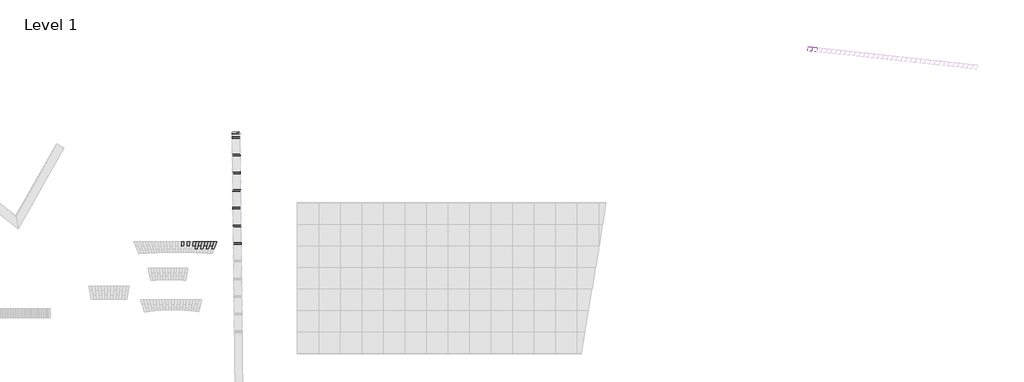
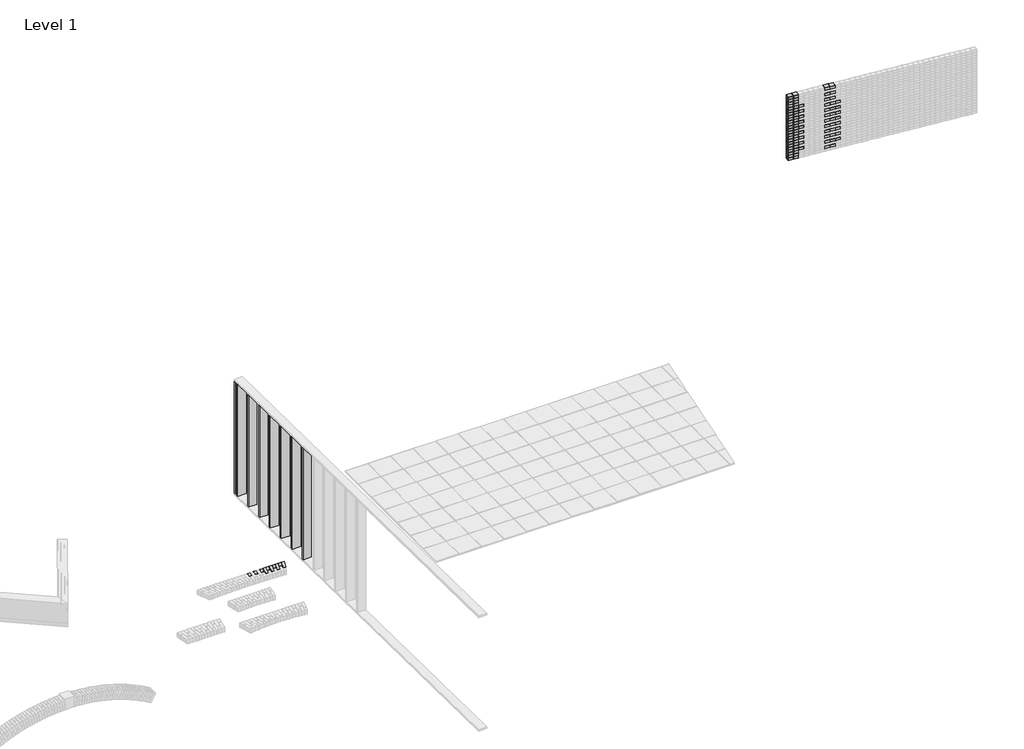
# One storey, part 11 of 18: 107 proxies.
"""IFC4 building model written with IfcOpenShell, lengths in millimetres."""

import ifcopenshell
import ifcopenshell.guid

model = None  # the IFC model being written
_history = None  # IfcOwnerHistory: only IFC2X3 demands one
_inside = {}  # id of a spatial element -> (the spatial element, [elements in it])
_under = {}  # id of a project, library or spatial element -> (it, [spatial elements below it])
_declared = {}  # id of a project -> (the project, [libraries it declares])
_typed = {}  # id of a type object -> (the type object, [elements of that type])
_made_of = {}  # id of a material, layer set ... -> (it, [elements and type objects made of it])


def new_model(schema):
    """Start an empty IFC model of exactly this schema.

    Asked for "IFC4X3", IfcOpenShell would pick the latest addendum, in which some entities
    have other attributes; the version numbers below select the first issue.
    IFC2X3 requires an IfcOwnerHistory on every rooted entity: one is made here for all.
    """
    global model, _history
    if schema == "IFC4X3":
        model = ifcopenshell.file(schema_version=(4, 3, 0, 0))
    else:
        model = ifcopenshell.file(schema=schema)
    _inside.clear()
    _under.clear()
    _declared.clear()
    _typed.clear()
    _made_of.clear()
    _history = None
    if model.schema == "IFC2X3":
        org = make("IfcOrganization", Name="unknown")
        user = make(
            "IfcPersonAndOrganization",
            ThePerson=make("IfcPerson", FamilyName="unknown"),
            TheOrganization=org,
        )
        app = make(
            "IfcApplication",
            ApplicationDeveloper=org,
            Version="unknown",
            ApplicationFullName="unknown",
            ApplicationIdentifier="unknown",
        )
        _history = make(
            "IfcOwnerHistory",
            OwningUser=user,
            OwningApplication=app,
            ChangeAction="ADDED",
            CreationDate=0,
        )
    return model


def make(cls, **values):
    """One entity of the class cls with the attributes given. An attribute that is None is left unset."""
    return model.create_entity(
        cls, **{name: value for name, value in values.items() if value is not None}
    )


def rooted(cls, **values):
    """An entity with a GlobalId (a new one), such as an element, a storey or a relation."""
    return make(cls, GlobalId=ifcopenshell.guid.new(), OwnerHistory=_history, **values)


def si_unit(unit_type, name, prefix=None):
    """IfcSIUnit, for example si_unit("LENGTHUNIT", "METRE", prefix="MILLI")."""
    return make("IfcSIUnit", UnitType=unit_type, Prefix=prefix, Name=name)


def assignment(units):
    """IfcUnitAssignment: the units of a project."""
    return None if units is None else make("IfcUnitAssignment", Units=units)


def point(xyz):
    """IfcCartesianPoint."""
    return None if xyz is None else make("IfcCartesianPoint", Coordinates=xyz)


def direction(xyz):
    """IfcDirection."""
    return None if xyz is None else make("IfcDirection", DirectionRatios=xyz)


def frame(location, z_axis=None, x_axis=None):
    """IfcAxis2Placement3D, a coordinate frame: its origin and axes. An axis left out is left unset."""
    return make(
        "IfcAxis2Placement3D",
        Location=point(location),
        Axis=direction(z_axis),
        RefDirection=direction(x_axis),
    )


def origin():
    """The frame at (0, 0, 0) with its axes left unset."""
    return frame((0.0, 0.0, 0.0))


def origin_with_axes():
    """The frame at (0, 0, 0) with the z axis (0, 0, 1) and the x axis (1, 0, 0) written out."""
    return frame((0.0, 0.0, 0.0), z_axis=(0.0, 0.0, 1.0), x_axis=(1.0, 0.0, 0.0))


def place(relative_to, where):
    """IfcLocalPlacement: puts the frame where relative to a parent placement (None: the world)."""
    return make(
        "IfcLocalPlacement", PlacementRelTo=relative_to, RelativePlacement=where
    )


def context(
    kind, dimensions, precision=None, world=None, true_north=None, identifier=None
):
    """IfcGeometricRepresentationContext, for example the 3D "Model" context."""
    return make(
        "IfcGeometricRepresentationContext",
        ContextIdentifier=identifier,
        ContextType=kind,
        CoordinateSpaceDimension=dimensions,
        Precision=precision,
        WorldCoordinateSystem=world,
        TrueNorth=true_north,
    )


def project(units=None, contexts=None):
    """IfcProject with its units and contexts."""
    return rooted(
        "IfcProject",
        Name="project",
        RepresentationContexts=contexts,
        UnitsInContext=assignment(units),
    )


def spatial(cls, under=None, at=None, **own):
    """A site, building, storey or space (cls), placed at a placement, below another one or the project."""
    s = rooted(cls, ObjectPlacement=at, **own)
    if under is not None:
        _under.setdefault(under.id(), (under, []))[1].append(s)
    return s


def polyline(points):
    """IfcPolyline through the points."""
    return make("IfcPolyline", Points=[point(p) for p in points])


def outline(outer, holes=None, kind="AREA"):
    """IfcArbitraryClosedProfileDef: a profile drawn as a closed curve; with holes, ...WithVoids."""
    if holes is None:
        return make("IfcArbitraryClosedProfileDef", ProfileType=kind, OuterCurve=outer)
    return make(
        "IfcArbitraryProfileDefWithVoids",
        ProfileType=kind,
        OuterCurve=outer,
        InnerCurves=holes,
    )


def extrude(swept, where, along, depth):
    """IfcExtrudedAreaSolid: the profile swept, set in the frame where, extruded along a direction by depth."""
    return make(
        "IfcExtrudedAreaSolid",
        SweptArea=swept,
        Position=where,
        ExtrudedDirection=direction(along),
        Depth=depth,
    )


def shape(context_of_items, identifier, shape_type, items):
    """IfcShapeRepresentation: the items that make up one representation, for example the "Body"."""
    return make(
        "IfcShapeRepresentation",
        ContextOfItems=context_of_items,
        RepresentationIdentifier=identifier,
        RepresentationType=shape_type,
        Items=items,
    )


def source(mapping_origin, context_of_items, identifier, shape_type, items):
    """IfcRepresentationMap: a shape defined once, which mapped items show again and again."""
    return make(
        "IfcRepresentationMap",
        MappingOrigin=mapping_origin,
        MappedRepresentation=shape(context_of_items, identifier, shape_type, items),
    )


def transform(
    local_origin,
    x_axis=None,
    y_axis=None,
    z_axis=None,
    scale=None,
    scale2=None,
    scale3=None,
    uniform=True,
):
    """IfcCartesianTransformationOperator3D, or its non-uniform kind. x_axis, y_axis, z_axis: its Axis1, 2, 3."""
    if uniform:
        return make(
            "IfcCartesianTransformationOperator3D",
            Axis1=direction(x_axis),
            Axis2=direction(y_axis),
            LocalOrigin=point(local_origin),
            Scale=scale,
            Axis3=direction(z_axis),
        )
    return make(
        "IfcCartesianTransformationOperator3DnonUniform",
        Axis1=direction(x_axis),
        Axis2=direction(y_axis),
        LocalOrigin=point(local_origin),
        Scale=scale,
        Axis3=direction(z_axis),
        Scale2=scale2,
        Scale3=scale3,
    )


def mapped(mapping_source, mapping_target):
    """IfcMappedItem: shows the shape of a source again, moved by a transform."""
    return make(
        "IfcMappedItem", MappingSource=mapping_source, MappingTarget=mapping_target
    )


def made_of(thing, what):
    """Note that an element or type object is made of a material, layer set ...; save() writes the relation."""
    if what is not None:
        _made_of.setdefault(what.id(), (what, []))[1].append(thing)
    return thing


def element(
    cls,
    number,
    at=None,
    inside=None,
    cuts=None,
    type_object=None,
    material=None,
    context=None,
    identifier="Body",
    shape_type=None,
    held_by="IfcProductDefinitionShape",
    body=None,
    shapes=None,
    **own,
):
    """One element of the class cls, such as IfcWall. Its Tag is "e" and its number.

    at: its placement. inside: the storey or other place that contains it. cuts: it is an
    opening in that element (IfcRelVoidsElement). A single representation is given by context,
    identifier, shape_type and body (its items); several are given by shapes. held_by: the class
    of the entity that holds the representations. save() writes the other relations.
    """
    e = rooted(cls, Tag="e%d" % number, ObjectPlacement=at, **own)
    if body is not None:
        shapes = [shape(context, identifier, shape_type, body)]
    if shapes is not None:
        e.Representation = make(held_by, Representations=shapes)
    if inside is not None:
        _inside.setdefault(inside.id(), (inside, []))[1].append(e)
    if cuts is not None:
        rooted(
            "IfcRelVoidsElement", RelatingBuildingElement=cuts, RelatedOpeningElement=e
        )
    if type_object is not None:
        _typed.setdefault(type_object.id(), (type_object, []))[1].append(e)
    return made_of(e, material)


def aggregate(whole, parts):
    """IfcRelAggregates: a whole, such as a stair, and the parts it consists of."""
    return rooted("IfcRelAggregates", RelatingObject=whole, RelatedObjects=parts)


def save(model, path):
    """Write the relations noted so far, then the file.

    IfcRelAggregates (storeys below a building ...), IfcRelContainedInSpatialStructure (elements
    in a storey), IfcRelDefinesByType, IfcRelAssociatesMaterial and IfcRelDeclares: one each for
    every whole, place, type object, material and project.
    """
    for whole, parts in _under.values():
        aggregate(whole, parts)
    for where, things in _inside.values():
        rooted(
            "IfcRelContainedInSpatialStructure",
            RelatedElements=things,
            RelatingStructure=where,
        )
    for kind, things in _typed.values():
        rooted("IfcRelDefinesByType", RelatedObjects=things, RelatingType=kind)
    for what, things in _made_of.values():
        rooted("IfcRelAssociatesMaterial", RelatedObjects=things, RelatingMaterial=what)
    for by, libraries in _declared.values():
        rooted("IfcRelDeclares", RelatingContext=by, RelatedDefinitions=libraries)
    model.write(path)


def proxy_00_gma_hout_184x38_1d2382f2(model_context):
    return source(origin(), model_context, "Body", "SweptSolid", [
        extrude(outline(polyline([(-19.0, 0.0), (19.0, 0.0), (19.0, -2617.0000001), (-19.0, -2617.0000001), (-19.0, 0.0)])), frame((-400.2270235, 19.0, -613.6855812), z_axis=(-0.67357883778224, 0.0, 0.7391153829355245), x_axis=(0.0, 1.0, 0.0)), (0.0, 0.0, 1.0), 184.0),
    ])


def proxy_00_gma_hout_38x184_71ec18f3(model_context):
    return source(origin(), model_context, "Body", "SweptSolid", [
        extrude(outline(polyline([(-19.0, 0.0), (19.0, 0.0), (19.0, -2617.0000001), (-19.0, -2617.0000001), (-19.0, 0.0)])), frame((-400.2270235, 19.0, -613.6855812), z_axis=(-0.6735788377822399, 0.0, 0.7391153829355245), x_axis=(0.0, 1.0, 0.0)), (0.0, 0.0, 1.0), 184.0),
    ])


def geel_a5fc7152(model_context):
    return source(origin(), model_context, "Body", "SweptSolid", [
        extrude(outline(polyline([(131.1871262, 51.8695461), (24.8461542, 24.0369432), (23.5801491, 28.8740117), (125.0840527, 55.4406095), (111.9430518, 105.6488784), (10.4391482, 79.0822806), (9.1731432, 83.919349), (115.5141152, 111.7519519), (131.1871262, 51.8695461)])), origin_with_axes(), (0.0, 0.0, 1.0), 95.0),
        extrude(outline(polyline([(111.9430518, 105.6488784), (125.0840527, 55.4406095), (23.5801491, 28.8740117), (10.4391482, 79.0822806), (111.9430518, 105.6488784)])), origin_with_axes(), (0.0, 0.0, 1.0), 100.0),
    ])


def geel_ff5a4212(model_context):
    return source(origin(), model_context, "Body", "SweptSolid", [
        extrude(outline(polyline([(24.8461542, 24.0369432), (9.1731432, 83.919349), (115.5141152, 111.7519519), (116.7801202, 106.9148835), (15.2762167, 80.3482856), (28.4172176, 30.1400167), (129.9211211, 56.7066146), (131.1871262, 51.8695461), (24.8461542, 24.0369432)])), origin_with_axes(), (0.0, 0.0, 1.0), 95.0),
        extrude(outline(polyline([(116.7801202, 106.9148835), (129.9211211, 56.7066146), (28.4172176, 30.1400167), (15.2762167, 80.3482856), (116.7801202, 106.9148835)])), origin_with_axes(), (0.0, 0.0, 1.0), 100.0),
    ])


def rood_14a66368(model_context):
    return source(origin(), model_context, "Body", "SweptSolid", [
        extrude(outline(polyline([(24.8461542, 24.0369432), (9.1731432, 83.919349), (115.5141152, 111.7519519), (131.1871262, 51.8695461), (24.8461542, 24.0369432)]), holes=[polyline([(125.0840527, 55.4406095), (111.9430518, 105.6488784), (15.2762167, 80.3482856), (28.4172176, 30.1400167), (125.0840527, 55.4406095)])]), origin_with_axes(), (0.0, 0.0, 1.0), 95.0),
        extrude(outline(polyline([(111.9430518, 105.6488784), (125.0840527, 55.4406095), (28.4172176, 30.1400167), (15.2762167, 80.3482856), (111.9430518, 105.6488784)])), origin_with_axes(), (0.0, 0.0, 1.0), 100.0),
    ])


def steen_boven_01e32946(model_context):
    return source(origin(), model_context, "Body", "SweptSolid", [
        extrude(outline(polyline([(141.1704134, 152.36343), (62.4529027, -8.187695), (10.0350866, 5.3211774), (84.0648392, 167.0564768), (141.1704134, 152.36343)])), origin_with_axes(), (0.0, 0.0, 1.0), 100.0),
    ])


def steen_boven_6e46f58c(model_context):
    return source(origin(), model_context, "Body", "SweptSolid", [
        extrude(outline(polyline([(143.5582911, 152.2686047), (60.0999612, -8.4277022), (7.3163998, 3.5526856), (86.0489792, 165.2920935), (143.5582911, 152.2686047)])), origin_with_axes(), (0.0, 0.0, 1.0), 100.0),
    ])


def steen_boven_eabcd001(model_context):
    return source(origin(), model_context, "Body", "SweptSolid", [
        extrude(outline(polyline([(146.1086958, 152.321622), (57.5952589, -8.8049317), (4.5075261, 1.71935), (88.2622432, 163.7549131), (146.1086958, 152.321622)])), origin_with_axes(), (0.0, 0.0, 1.0), 100.0),
    ])


def steen_boven_7310186c(model_context):
    return source(origin(), model_context, "Body", "SweptSolid", [
        extrude(outline(polyline([(148.8055175, 152.5156886), (54.9522509, -9.3122663), (1.614426, -0.1736166), (90.6804944, 162.4360672), (148.8055175, 152.5156886)])), origin_with_axes(), (0.0, 0.0, 1.0), 100.0),
    ])


def steen_boven_9bb71775(model_context):
    return source(origin(), model_context, "Body", "SweptSolid", [
        extrude(outline(polyline([(111.9849233, 118.6347443), (90.2344792, 23.3760955), (33.8999775, 23.0709028), (53.0204132, 118.2901143), (111.9849233, 118.6347443)])), origin_with_axes(), (0.0, 0.0, 1.0), 100.0),
    ])


def steen_boven_9cbfec4d(model_context):
    return source(origin(), model_context, "Body", "SweptSolid", [
        extrude(outline(polyline([(113.9568566, 118.7889283), (88.4390091, 23.0223042), (32.1209988, 21.8380681), (55.0050159, 117.5190081), (113.9568566, 118.7889283)])), origin_with_axes(), (0.0, 0.0, 1.0), 100.0),
    ])


def steen_boven_ecc8bb5a(model_context):
    return source(origin(), model_context, "Body", "SweptSolid", [
        extrude(outline(polyline([(115.9629985, 119.0094516), (86.6063002, 22.6045748), (30.3176515, 20.5836998), (57.0367025, 116.8591339), (115.9629985, 119.0094516)])), origin_with_axes(), (0.0, 0.0, 1.0), 100.0),
    ])


def steen_boven_26140218(model_context):
    return source(origin(), model_context, "Body", "SweptSolid", [
        extrude(outline(polyline([(106.3172402, 118.6145349), (95.374274, 24.0083503), (39.0907656, 26.6225769), (47.4149135, 121.3436608), (106.3172402, 118.6145349)])), origin_with_axes(), (0.0, 0.0, 1.0), 100.0),
    ])


def steen_boven_4abb9939(model_context):
    return source(origin(), model_context, "Body", "SweptSolid", [
        extrude(outline(polyline([(108.1602922, 118.5428629), (93.704652, 23.8737179), (37.3847868, 25.4648208), (49.2179184, 120.1947689), (108.1602922, 118.5428629)])), origin_with_axes(), (0.0, 0.0, 1.0), 100.0),
    ])


def steen_boven_6d657369(model_context):
    return source(origin(), model_context, "Body", "SweptSolid", [
        extrude(outline(polyline([(110.0512234, 118.5512029), (91.9904937, 23.66143), (35.6545533, 24.2803953), (51.0890541, 119.1795406), (110.0512234, 118.5512029)])), origin_with_axes(), (0.0, 0.0, 1.0), 100.0),
    ])


model = new_model("IFC4")

# Units and contexts
model_context = context("Model", 3, world=origin())
ifc_project = project(units=[si_unit("LENGTHUNIT", "METRE", prefix="MILLI")], contexts=[model_context])

# Site, building, storey
site = spatial("IfcSite", under=ifc_project)
building = spatial("IfcBuilding", under=site)
storey = spatial("IfcBuildingStorey", under=building, Name="Level 1", Elevation=0.0)

# Proxies
placement = place(None, origin())
proxy_00_gma_hout_184x38_shape = proxy_00_gma_hout_184x38_1d2382f2(model_context)
element("IfcBuildingElementProxy", 1, Name="00_GMA_hout : 184x38", ObjectType="00_GMA_hout : 184x38", at=placement, inside=storey, context=model_context, shape_type="MappedRepresentation", body=[
    mapped(proxy_00_gma_hout_184x38_shape, transform((-4279.0312737, -6270.7891061, 754.1795702), x_axis=(-0.6735355593090224, -0.007635512710727629, 0.7391153829355245), y_axis=(0.011335737232879188, -0.9999357484665639, 0.0), z_axis=(0.7390678936387847, 0.008378417765735984, 0.67357883778224))),
])
proxy_00_gma_hout_38x184_shape = proxy_00_gma_hout_38x184_71ec18f3(model_context)
element("IfcBuildingElementProxy", 2, Name="00_GMA_hout : 38x184", ObjectType="00_GMA_hout : 38x184", at=placement, inside=storey, context=model_context, shape_type="MappedRepresentation", body=[
    mapped(proxy_00_gma_hout_38x184_shape, transform((-4250.0117864, -8830.6246222, 754.1795702), x_axis=(-0.6735355593090224, -0.007635512710727629, 0.7391153829355245), y_axis=(0.011335737232879188, -0.9999357484665639, 0.0), z_axis=(0.7390678936387847, 0.008378417765735984, 0.67357883778224))),
])
element("IfcBuildingElementProxy", 3, Name="00_GMA_hout : 38x184", ObjectType="00_GMA_hout : 38x184", at=placement, inside=storey, context=model_context, shape_type="MappedRepresentation", body=[
    mapped(proxy_00_gma_hout_38x184_shape, transform((-4254.6594386, -8420.6509653, 754.1795702), x_axis=(-0.6735355593090224, -0.007635512710727629, 0.7391153829355245), y_axis=(0.011335737232879188, -0.9999357484665639, 0.0), z_axis=(0.7390678936387847, 0.008378417765735984, 0.67357883778224))),
])
element("IfcBuildingElementProxy", 4, Name="00_GMA_hout : 38x184", ObjectType="00_GMA_hout : 38x184", at=placement, inside=storey, context=model_context, shape_type="MappedRepresentation", body=[
    mapped(proxy_00_gma_hout_38x184_shape, transform((-4259.3070909, -8010.6773084, 754.1795702), x_axis=(-0.6735355593090224, -0.007635512710727629, 0.7391153829355245), y_axis=(0.011335737232879188, -0.9999357484665639, 0.0), z_axis=(0.7390678936387847, 0.008378417765735984, 0.67357883778224))),
])
element("IfcBuildingElementProxy", 5, Name="00_GMA_hout : 38x184", ObjectType="00_GMA_hout : 38x184", at=placement, inside=storey, context=model_context, shape_type="MappedRepresentation", body=[
    mapped(proxy_00_gma_hout_38x184_shape, transform((-4263.9547432, -7600.7036515, 754.1795702), x_axis=(-0.6735355593090224, -0.007635512710727629, 0.7391153829355245), y_axis=(0.011335737232879188, -0.9999357484665639, 0.0), z_axis=(0.7390678936387847, 0.008378417765735984, 0.67357883778224))),
])
element("IfcBuildingElementProxy", 6, Name="00_GMA_hout : 38x184", ObjectType="00_GMA_hout : 38x184", at=placement, inside=storey, context=model_context, shape_type="MappedRepresentation", body=[
    mapped(proxy_00_gma_hout_38x184_shape, transform((-4268.6023954, -7190.7299947, 754.1795702), x_axis=(-0.6735355593090224, -0.007635512710727629, 0.7391153829355245), y_axis=(0.011335737232879188, -0.9999357484665639, 0.0), z_axis=(0.7390678936387847, 0.008378417765735984, 0.67357883778224))),
])
element("IfcBuildingElementProxy", 7, Name="00_GMA_hout : 38x184", ObjectType="00_GMA_hout : 38x184", at=placement, inside=storey, context=model_context, shape_type="MappedRepresentation", body=[
    mapped(proxy_00_gma_hout_38x184_shape, transform((-4273.2500477, -6780.7563378, 754.1795702), x_axis=(-0.6735355593090224, -0.007635512710727629, 0.7391153829355245), y_axis=(0.011335737232879188, -0.9999357484665639, 0.0), z_axis=(0.7390678936387847, 0.008378417765735984, 0.67357883778224))),
])
element("IfcBuildingElementProxy", 8, Name="00_GMA_hout : 38x184", ObjectType="00_GMA_hout : 38x184", at=placement, inside=storey, context=model_context, shape_type="MappedRepresentation", body=[
    mapped(proxy_00_gma_hout_38x184_shape, transform((-4277.8977, -6370.7826809, 754.1795702), x_axis=(-0.6735355593090224, -0.007635512710727629, 0.7391153829355245), y_axis=(0.011335737232879188, -0.9999357484665639, 0.0), z_axis=(0.7390678936387847, 0.008378417765735984, 0.67357883778224))),
])
geel_shape = geel_a5fc7152(model_context)
element("IfcBuildingElementProxy", 9, Name="Geel", ObjectType="Geel", at=placement, inside=storey, context=model_context, shape_type="MappedRepresentation", body=[
    mapped(geel_shape, transform((8877.089595, -4276.2647708, 2168.7358475), x_axis=(0.9617275503729374, -0.10473475661477244, -0.25320100633787673), y_axis=(0.25171277368869216, -0.02741220845642972, 0.9674136914420255), z_axis=(-0.10826263628609079, -0.9941223272738551, 0.0))),
])
element("IfcBuildingElementProxy", 10, Name="Geel", ObjectType="Geel", at=placement, inside=storey, context=model_context, shape_type="MappedRepresentation", body=[
    mapped(geel_shape, transform((9642.0276443, -4359.5686133, 2168.7358475), x_axis=(0.9617275503729374, -0.1047347566147725, -0.25320100633787673), y_axis=(0.25171277368869216, -0.02741220845642974, 0.9674136914420255), z_axis=(-0.10826263628609081, -0.9941223272738551, 0.0))),
])
element("IfcBuildingElementProxy", 11, Name="Geel", ObjectType="Geel", at=placement, inside=storey, context=model_context, shape_type="MappedRepresentation", body=[
    mapped(geel_shape, transform((8877.089595, -4276.2647708, 2292.5348104), x_axis=(0.9617275503729374, -0.10473475661477244, -0.25320100633787673), y_axis=(0.25171277368869216, -0.02741220845642972, 0.9674136914420255), z_axis=(-0.10826263628609079, -0.9941223272738551, 0.0))),
])
element("IfcBuildingElementProxy", 12, Name="Geel", ObjectType="Geel", at=placement, inside=storey, context=model_context, shape_type="MappedRepresentation", body=[
    mapped(geel_shape, transform((9642.0276443, -4359.5686133, 2292.5348104), x_axis=(0.9617275503729374, -0.1047347566147725, -0.25320100633787673), y_axis=(0.25171277368869216, -0.02741220845642974, 0.9674136914420255), z_axis=(-0.10826263628609081, -0.9941223272738551, 0.0))),
])
element("IfcBuildingElementProxy", 13, Name="Geel", ObjectType="Geel", at=placement, inside=storey, context=model_context, shape_type="MappedRepresentation", body=[
    mapped(geel_shape, transform((8877.089595, -4276.2647708, 2416.3337732), x_axis=(0.9617275503729384, -0.10473475661477256, -0.25320100633787307), y_axis=(0.25171277368868855, -0.02741220845642932, 0.9674136914420265), z_axis=(-0.10826263628609077, -0.994122327273855, 0.0))),
])
element("IfcBuildingElementProxy", 14, Name="Geel", ObjectType="Geel", at=placement, inside=storey, context=model_context, shape_type="MappedRepresentation", body=[
    mapped(geel_shape, transform((9642.0276443, -4359.5686133, 2416.3337732), x_axis=(0.9617275503729384, -0.1047347566147726, -0.25320100633787307), y_axis=(0.25171277368868855, -0.02741220845642934, 0.9674136914420265), z_axis=(-0.10826263628609081, -0.994122327273855, 0.0))),
])
element("IfcBuildingElementProxy", 15, Name="Geel", ObjectType="Geel", at=placement, inside=storey, context=model_context, shape_type="MappedRepresentation", body=[
    mapped(geel_shape, transform((8877.089595, -4276.2647708, 2540.132736), x_axis=(0.9617275503729374, -0.10473475661477244, -0.25320100633787673), y_axis=(0.25171277368869216, -0.02741220845642972, 0.9674136914420255), z_axis=(-0.10826263628609079, -0.9941223272738551, 0.0))),
])
element("IfcBuildingElementProxy", 16, Name="Geel", ObjectType="Geel", at=placement, inside=storey, context=model_context, shape_type="MappedRepresentation", body=[
    mapped(geel_shape, transform((9642.0276443, -4359.5686133, 2540.132736), x_axis=(0.9617275503729374, -0.1047347566147725, -0.25320100633787673), y_axis=(0.25171277368869216, -0.02741220845642974, 0.9674136914420255), z_axis=(-0.10826263628609081, -0.9941223272738551, 0.0))),
])
element("IfcBuildingElementProxy", 17, Name="Geel", ObjectType="Geel", at=placement, inside=storey, context=model_context, shape_type="MappedRepresentation", body=[
    mapped(geel_shape, transform((8877.089595, -4276.2647708, 2663.9316989), x_axis=(0.9617275503729374, -0.10473475661477244, -0.25320100633787673), y_axis=(0.25171277368869216, -0.02741220845642972, 0.9674136914420255), z_axis=(-0.10826263628609079, -0.9941223272738551, 0.0))),
])
element("IfcBuildingElementProxy", 18, Name="Geel", ObjectType="Geel", at=placement, inside=storey, context=model_context, shape_type="MappedRepresentation", body=[
    mapped(geel_shape, transform((9642.0276443, -4359.5686133, 2663.9316989), x_axis=(0.9617275503729374, -0.1047347566147725, -0.25320100633787673), y_axis=(0.25171277368869216, -0.02741220845642974, 0.9674136914420255), z_axis=(-0.10826263628609081, -0.9941223272738551, 0.0))),
])
element("IfcBuildingElementProxy", 19, Name="Geel", ObjectType="Geel", at=placement, inside=storey, context=model_context, shape_type="MappedRepresentation", body=[
    mapped(geel_shape, transform((8877.089595, -4276.2647708, 2787.7306617), x_axis=(0.9617275503729374, -0.10473475661477244, -0.25320100633787673), y_axis=(0.25171277368869216, -0.02741220845642972, 0.9674136914420255), z_axis=(-0.10826263628609079, -0.9941223272738551, 0.0))),
])
element("IfcBuildingElementProxy", 20, Name="Geel", ObjectType="Geel", at=placement, inside=storey, context=model_context, shape_type="MappedRepresentation", body=[
    mapped(geel_shape, transform((9642.0276443, -4359.5686133, 2787.7306617), x_axis=(0.9617275503729374, -0.1047347566147725, -0.25320100633787673), y_axis=(0.25171277368869216, -0.02741220845642974, 0.9674136914420255), z_axis=(-0.10826263628609081, -0.9941223272738551, 0.0))),
])
element("IfcBuildingElementProxy", 21, Name="Geel", ObjectType="Geel", at=placement, inside=storey, context=model_context, shape_type="MappedRepresentation", body=[
    mapped(geel_shape, transform((8877.089595, -4276.2647708, 2911.5296245), x_axis=(0.9617275503729374, -0.10473475661477244, -0.25320100633787673), y_axis=(0.25171277368869216, -0.02741220845642972, 0.9674136914420255), z_axis=(-0.10826263628609079, -0.9941223272738551, 0.0))),
])
element("IfcBuildingElementProxy", 22, Name="Geel", ObjectType="Geel", at=placement, inside=storey, context=model_context, shape_type="MappedRepresentation", body=[
    mapped(geel_shape, transform((9642.0276443, -4359.5686133, 2911.5296245), x_axis=(0.9617275503729374, -0.1047347566147725, -0.25320100633787673), y_axis=(0.25171277368869216, -0.02741220845642974, 0.9674136914420255), z_axis=(-0.10826263628609081, -0.9941223272738551, 0.0))),
])
element("IfcBuildingElementProxy", 23, Name="Geel", ObjectType="Geel", at=placement, inside=storey, context=model_context, shape_type="MappedRepresentation", body=[
    mapped(geel_shape, transform((8877.089595, -4276.2647708, 3035.3285874), x_axis=(0.9617275503729374, -0.10473475661477244, -0.25320100633787673), y_axis=(0.25171277368869216, -0.02741220845642972, 0.9674136914420255), z_axis=(-0.10826263628609079, -0.9941223272738551, 0.0))),
])
element("IfcBuildingElementProxy", 24, Name="Geel", ObjectType="Geel", at=placement, inside=storey, context=model_context, shape_type="MappedRepresentation", body=[
    mapped(geel_shape, transform((9642.0276443, -4359.5686133, 3035.3285874), x_axis=(0.9617275503729374, -0.1047347566147725, -0.25320100633787673), y_axis=(0.25171277368869216, -0.02741220845642974, 0.9674136914420255), z_axis=(-0.10826263628609081, -0.9941223272738551, 0.0))),
])
element("IfcBuildingElementProxy", 25, Name="Geel", ObjectType="Geel", at=placement, inside=storey, context=model_context, shape_type="MappedRepresentation", body=[
    mapped(geel_shape, transform((8877.089595, -4276.2647708, 3159.1275502), x_axis=(0.9617275503729374, -0.10473475661477244, -0.25320100633787673), y_axis=(0.25171277368869216, -0.02741220845642972, 0.9674136914420255), z_axis=(-0.10826263628609079, -0.9941223272738551, 0.0))),
])
element("IfcBuildingElementProxy", 26, Name="Geel", ObjectType="Geel", at=placement, inside=storey, context=model_context, shape_type="MappedRepresentation", body=[
    mapped(geel_shape, transform((9642.0276443, -4359.5686133, 3159.1275502), x_axis=(0.9617275503729374, -0.1047347566147725, -0.25320100633787673), y_axis=(0.25171277368869216, -0.02741220845642974, 0.9674136914420255), z_axis=(-0.10826263628609081, -0.9941223272738551, 0.0))),
])
element("IfcBuildingElementProxy", 27, Name="Geel", ObjectType="Geel", at=placement, inside=storey, context=model_context, shape_type="MappedRepresentation", body=[
    mapped(geel_shape, transform((8877.089595, -4276.2647708, 3282.926513), x_axis=(0.9617275503729374, -0.10473475661477244, -0.25320100633787673), y_axis=(0.25171277368869216, -0.02741220845642972, 0.9674136914420255), z_axis=(-0.10826263628609079, -0.9941223272738551, 0.0))),
])
element("IfcBuildingElementProxy", 28, Name="Geel", ObjectType="Geel", at=placement, inside=storey, context=model_context, shape_type="MappedRepresentation", body=[
    mapped(geel_shape, transform((9642.0276443, -4359.5686133, 3282.926513), x_axis=(0.9617275503729374, -0.1047347566147725, -0.25320100633787673), y_axis=(0.25171277368869216, -0.02741220845642974, 0.9674136914420255), z_axis=(-0.10826263628609081, -0.9941223272738551, 0.0))),
])
element("IfcBuildingElementProxy", 29, Name="Geel", ObjectType="Geel", at=placement, inside=storey, context=model_context, shape_type="MappedRepresentation", body=[
    mapped(geel_shape, transform((8877.089595, -4276.2647708, 3406.7254759), x_axis=(0.9617275503729374, -0.10473475661477244, -0.25320100633787673), y_axis=(0.25171277368869216, -0.02741220845642972, 0.9674136914420255), z_axis=(-0.10826263628609079, -0.9941223272738551, 0.0))),
])
element("IfcBuildingElementProxy", 30, Name="Geel", ObjectType="Geel", at=placement, inside=storey, context=model_context, shape_type="MappedRepresentation", body=[
    mapped(geel_shape, transform((9642.0276443, -4359.5686133, 3406.7254759), x_axis=(0.9617275503729374, -0.1047347566147725, -0.25320100633787673), y_axis=(0.25171277368869216, -0.02741220845642974, 0.9674136914420255), z_axis=(-0.10826263628609081, -0.9941223272738551, 0.0))),
])
element("IfcBuildingElementProxy", 31, Name="Geel", ObjectType="Geel", at=placement, inside=storey, context=model_context, shape_type="MappedRepresentation", body=[
    mapped(geel_shape, transform((8877.089595, -4276.2647708, 2044.9368847), x_axis=(0.9617275503729384, -0.10473475661477256, -0.25320100633787307), y_axis=(0.25171277368868855, -0.02741220845642932, 0.9674136914420265), z_axis=(-0.10826263628609077, -0.994122327273855, 0.0))),
])
element("IfcBuildingElementProxy", 32, Name="Geel", ObjectType="Geel", at=placement, inside=storey, context=model_context, shape_type="MappedRepresentation", body=[
    mapped(geel_shape, transform((9642.0276443, -4359.5686133, 2044.9368847), x_axis=(0.9617275503729384, -0.1047347566147726, -0.25320100633787307), y_axis=(0.25171277368868855, -0.02741220845642934, 0.9674136914420265), z_axis=(-0.10826263628609081, -0.994122327273855, 0.0))),
])
element("IfcBuildingElementProxy", 33, Name="Geel", ObjectType="Geel", at=placement, inside=storey, context=model_context, shape_type="MappedRepresentation", body=[
    mapped(geel_shape, transform((9095.6433234, -4300.0658686, 2168.7358475), x_axis=(0.9617275503729401, -0.10473475661476903, -0.2532010063378687), y_axis=(0.2517127736886843, -0.02741220845642789, 0.9674136914420278), z_axis=(-0.108262636286087, -0.9941223272738555, 0.0))),
])
element("IfcBuildingElementProxy", 34, Name="Geel", ObjectType="Geel", at=placement, inside=storey, context=model_context, shape_type="MappedRepresentation", body=[
    mapped(geel_shape, transform((9860.5813726, -4383.3697112, 2168.7358475), x_axis=(0.9617275503729372, -0.1047347566147745, -0.2532010063378768), y_axis=(0.2517127736886921, -0.02741220845643024, 0.9674136914420256), z_axis=(-0.10826263628609285, -0.9941223272738547, 0.0))),
])
element("IfcBuildingElementProxy", 35, Name="Geel", ObjectType="Geel", at=placement, inside=storey, context=model_context, shape_type="MappedRepresentation", body=[
    mapped(geel_shape, transform((9095.6433234, -4300.0658686, 2292.5348104), x_axis=(0.9617275503729401, -0.10473475661476903, -0.2532010063378687), y_axis=(0.2517127736886843, -0.02741220845642789, 0.9674136914420278), z_axis=(-0.108262636286087, -0.9941223272738555, 0.0))),
])
element("IfcBuildingElementProxy", 36, Name="Geel", ObjectType="Geel", at=placement, inside=storey, context=model_context, shape_type="MappedRepresentation", body=[
    mapped(geel_shape, transform((9860.5813726, -4383.3697112, 2292.5348104), x_axis=(0.9617275503729372, -0.1047347566147745, -0.2532010063378768), y_axis=(0.2517127736886921, -0.02741220845643024, 0.9674136914420256), z_axis=(-0.10826263628609285, -0.9941223272738547, 0.0))),
])
element("IfcBuildingElementProxy", 37, Name="Geel", ObjectType="Geel", at=placement, inside=storey, context=model_context, shape_type="MappedRepresentation", body=[
    mapped(geel_shape, transform((9095.6433234, -4300.0658686, 2416.3337732), x_axis=(0.961727550372941, -0.10473475661476911, -0.2532010063378651), y_axis=(0.2517127736886807, -0.0274122084564275, 0.9674136914420286), z_axis=(-0.10826263628608698, -0.9941223272738555, 0.0))),
])
element("IfcBuildingElementProxy", 38, Name="Geel", ObjectType="Geel", at=placement, inside=storey, context=model_context, shape_type="MappedRepresentation", body=[
    mapped(geel_shape, transform((9860.5813726, -4383.3697112, 2416.3337732), x_axis=(0.9617275503729381, -0.10473475661477456, -0.2532010063378731), y_axis=(0.2517127736886886, -0.02741220845642988, 0.9674136914420264), z_axis=(-0.10826263628609287, -0.9941223272738549, 0.0))),
])
element("IfcBuildingElementProxy", 39, Name="Geel", ObjectType="Geel", at=placement, inside=storey, context=model_context, shape_type="MappedRepresentation", body=[
    mapped(geel_shape, transform((9095.6433234, -4300.0658686, 2540.132736), x_axis=(0.9617275503729401, -0.10473475661476903, -0.2532010063378687), y_axis=(0.2517127736886843, -0.02741220845642789, 0.9674136914420278), z_axis=(-0.108262636286087, -0.9941223272738555, 0.0))),
])
element("IfcBuildingElementProxy", 40, Name="Geel", ObjectType="Geel", at=placement, inside=storey, context=model_context, shape_type="MappedRepresentation", body=[
    mapped(geel_shape, transform((9860.5813726, -4383.3697112, 2540.132736), x_axis=(0.9617275503729372, -0.1047347566147745, -0.2532010063378768), y_axis=(0.2517127736886921, -0.02741220845643024, 0.9674136914420256), z_axis=(-0.10826263628609285, -0.9941223272738547, 0.0))),
])
element("IfcBuildingElementProxy", 41, Name="Geel", ObjectType="Geel", at=placement, inside=storey, context=model_context, shape_type="MappedRepresentation", body=[
    mapped(geel_shape, transform((9095.6433234, -4300.0658686, 2663.9316989), x_axis=(0.9617275503729401, -0.10473475661476903, -0.2532010063378687), y_axis=(0.2517127736886843, -0.02741220845642789, 0.9674136914420278), z_axis=(-0.108262636286087, -0.9941223272738555, 0.0))),
])
element("IfcBuildingElementProxy", 42, Name="Geel", ObjectType="Geel", at=placement, inside=storey, context=model_context, shape_type="MappedRepresentation", body=[
    mapped(geel_shape, transform((9860.5813726, -4383.3697112, 2663.9316989), x_axis=(0.9617275503729372, -0.1047347566147745, -0.2532010063378768), y_axis=(0.2517127736886921, -0.02741220845643024, 0.9674136914420256), z_axis=(-0.10826263628609285, -0.9941223272738547, 0.0))),
])
element("IfcBuildingElementProxy", 43, Name="Geel", ObjectType="Geel", at=placement, inside=storey, context=model_context, shape_type="MappedRepresentation", body=[
    mapped(geel_shape, transform((9095.6433234, -4300.0658686, 2787.7306617), x_axis=(0.9617275503729401, -0.10473475661476903, -0.2532010063378687), y_axis=(0.2517127736886843, -0.02741220845642789, 0.9674136914420278), z_axis=(-0.108262636286087, -0.9941223272738555, 0.0))),
])
element("IfcBuildingElementProxy", 44, Name="Geel", ObjectType="Geel", at=placement, inside=storey, context=model_context, shape_type="MappedRepresentation", body=[
    mapped(geel_shape, transform((9860.5813726, -4383.3697112, 2787.7306617), x_axis=(0.9617275503729372, -0.1047347566147745, -0.2532010063378768), y_axis=(0.2517127736886921, -0.02741220845643024, 0.9674136914420256), z_axis=(-0.10826263628609285, -0.9941223272738547, 0.0))),
])
element("IfcBuildingElementProxy", 45, Name="Geel", ObjectType="Geel", at=placement, inside=storey, context=model_context, shape_type="MappedRepresentation", body=[
    mapped(geel_shape, transform((9095.6433234, -4300.0658686, 2911.5296245), x_axis=(0.9617275503729401, -0.10473475661476903, -0.2532010063378687), y_axis=(0.2517127736886843, -0.02741220845642789, 0.9674136914420278), z_axis=(-0.108262636286087, -0.9941223272738555, 0.0))),
])
element("IfcBuildingElementProxy", 46, Name="Geel", ObjectType="Geel", at=placement, inside=storey, context=model_context, shape_type="MappedRepresentation", body=[
    mapped(geel_shape, transform((9860.5813726, -4383.3697112, 2911.5296245), x_axis=(0.9617275503729372, -0.1047347566147745, -0.2532010063378768), y_axis=(0.2517127736886921, -0.02741220845643024, 0.9674136914420256), z_axis=(-0.10826263628609285, -0.9941223272738547, 0.0))),
])
element("IfcBuildingElementProxy", 47, Name="Geel", ObjectType="Geel", at=placement, inside=storey, context=model_context, shape_type="MappedRepresentation", body=[
    mapped(geel_shape, transform((9095.6433234, -4300.0658686, 3035.3285874), x_axis=(0.9617275503729401, -0.10473475661476903, -0.2532010063378687), y_axis=(0.2517127736886843, -0.02741220845642789, 0.9674136914420278), z_axis=(-0.108262636286087, -0.9941223272738555, 0.0))),
])
element("IfcBuildingElementProxy", 48, Name="Geel", ObjectType="Geel", at=placement, inside=storey, context=model_context, shape_type="MappedRepresentation", body=[
    mapped(geel_shape, transform((9860.5813726, -4383.3697112, 3035.3285874), x_axis=(0.9617275503729372, -0.1047347566147745, -0.2532010063378768), y_axis=(0.2517127736886921, -0.02741220845643024, 0.9674136914420256), z_axis=(-0.10826263628609285, -0.9941223272738547, 0.0))),
])
element("IfcBuildingElementProxy", 49, Name="Geel", ObjectType="Geel", at=placement, inside=storey, context=model_context, shape_type="MappedRepresentation", body=[
    mapped(geel_shape, transform((9095.6433234, -4300.0658686, 3159.1275502), x_axis=(0.9617275503729401, -0.10473475661476903, -0.2532010063378687), y_axis=(0.2517127736886843, -0.02741220845642789, 0.9674136914420278), z_axis=(-0.108262636286087, -0.9941223272738555, 0.0))),
])
geel_2_shape = geel_ff5a4212(model_context)
element("IfcBuildingElementProxy", 50, Name="Geel", ObjectType="Geel", at=placement, inside=storey, context=model_context, shape_type="MappedRepresentation", body=[
    mapped(geel_2_shape, transform((8986.3664592, -4288.1653197, 2168.7358475), x_axis=(0.9617275503729374, -0.10473475661477352, -0.25320100633787673), y_axis=(0.2517127736886921, -0.02741220845642999, 0.9674136914420257), z_axis=(-0.10826263628609187, -0.9941223272738549, 0.0))),
])
element("IfcBuildingElementProxy", 51, Name="Geel", ObjectType="Geel", at=placement, inside=storey, context=model_context, shape_type="MappedRepresentation", body=[
    mapped(geel_2_shape, transform((9751.3045085, -4371.4691622, 2168.7358475), x_axis=(0.9617275503729374, -0.1047347566147725, -0.25320100633787673), y_axis=(0.25171277368869216, -0.02741220845642974, 0.9674136914420255), z_axis=(-0.10826263628609081, -0.9941223272738551, 0.0))),
])
element("IfcBuildingElementProxy", 52, Name="Geel", ObjectType="Geel", at=placement, inside=storey, context=model_context, shape_type="MappedRepresentation", body=[
    mapped(geel_2_shape, transform((8986.3664592, -4288.1653197, 2292.5348104), x_axis=(0.9617275503729374, -0.10473475661477352, -0.25320100633787673), y_axis=(0.2517127736886921, -0.02741220845642999, 0.9674136914420257), z_axis=(-0.10826263628609187, -0.9941223272738549, 0.0))),
])
element("IfcBuildingElementProxy", 53, Name="Geel", ObjectType="Geel", at=placement, inside=storey, context=model_context, shape_type="MappedRepresentation", body=[
    mapped(geel_2_shape, transform((9751.3045085, -4371.4691622, 2292.5348104), x_axis=(0.9617275503729374, -0.1047347566147725, -0.25320100633787673), y_axis=(0.25171277368869216, -0.02741220845642974, 0.9674136914420255), z_axis=(-0.10826263628609081, -0.9941223272738551, 0.0))),
])
element("IfcBuildingElementProxy", 54, Name="Geel", ObjectType="Geel", at=placement, inside=storey, context=model_context, shape_type="MappedRepresentation", body=[
    mapped(geel_2_shape, transform((8986.3664592, -4288.1653197, 2416.3337732), x_axis=(0.9617275503729383, -0.1047347566147736, -0.25320100633787307), y_axis=(0.2517127736886885, -0.027412208456429603, 0.9674136914420265), z_axis=(-0.10826263628609187, -0.9941223272738549, 0.0))),
])
element("IfcBuildingElementProxy", 55, Name="Geel", ObjectType="Geel", at=placement, inside=storey, context=model_context, shape_type="MappedRepresentation", body=[
    mapped(geel_2_shape, transform((9751.3045085, -4371.4691622, 2416.3337732), x_axis=(0.9617275503729384, -0.1047347566147726, -0.25320100633787307), y_axis=(0.25171277368868855, -0.02741220845642934, 0.9674136914420265), z_axis=(-0.10826263628609081, -0.994122327273855, 0.0))),
])
element("IfcBuildingElementProxy", 56, Name="Geel", ObjectType="Geel", at=placement, inside=storey, context=model_context, shape_type="MappedRepresentation", body=[
    mapped(geel_2_shape, transform((8986.3664592, -4288.1653197, 2540.132736), x_axis=(0.9617275503729374, -0.10473475661477352, -0.25320100633787673), y_axis=(0.2517127736886921, -0.02741220845642999, 0.9674136914420257), z_axis=(-0.10826263628609187, -0.9941223272738549, 0.0))),
])
element("IfcBuildingElementProxy", 57, Name="Geel", ObjectType="Geel", at=placement, inside=storey, context=model_context, shape_type="MappedRepresentation", body=[
    mapped(geel_2_shape, transform((9751.3045085, -4371.4691622, 2540.132736), x_axis=(0.9617275503729374, -0.1047347566147725, -0.25320100633787673), y_axis=(0.25171277368869216, -0.02741220845642974, 0.9674136914420255), z_axis=(-0.10826263628609081, -0.9941223272738551, 0.0))),
])
element("IfcBuildingElementProxy", 58, Name="Geel", ObjectType="Geel", at=placement, inside=storey, context=model_context, shape_type="MappedRepresentation", body=[
    mapped(geel_2_shape, transform((8986.3664592, -4288.1653197, 2663.9316989), x_axis=(0.9617275503729374, -0.10473475661477352, -0.25320100633787673), y_axis=(0.2517127736886921, -0.02741220845642999, 0.9674136914420257), z_axis=(-0.10826263628609187, -0.9941223272738549, 0.0))),
])
element("IfcBuildingElementProxy", 59, Name="Geel", ObjectType="Geel", at=placement, inside=storey, context=model_context, shape_type="MappedRepresentation", body=[
    mapped(geel_2_shape, transform((9751.3045085, -4371.4691622, 2663.9316989), x_axis=(0.9617275503729374, -0.1047347566147725, -0.25320100633787673), y_axis=(0.25171277368869216, -0.02741220845642974, 0.9674136914420255), z_axis=(-0.10826263628609081, -0.9941223272738551, 0.0))),
])
element("IfcBuildingElementProxy", 60, Name="Geel", ObjectType="Geel", at=placement, inside=storey, context=model_context, shape_type="MappedRepresentation", body=[
    mapped(geel_2_shape, transform((8986.3664592, -4288.1653197, 2787.7306617), x_axis=(0.9617275503729374, -0.10473475661477352, -0.25320100633787673), y_axis=(0.2517127736886921, -0.02741220845642999, 0.9674136914420257), z_axis=(-0.10826263628609187, -0.9941223272738549, 0.0))),
])
element("IfcBuildingElementProxy", 61, Name="Geel", ObjectType="Geel", at=placement, inside=storey, context=model_context, shape_type="MappedRepresentation", body=[
    mapped(geel_2_shape, transform((9751.3045085, -4371.4691622, 2787.7306617), x_axis=(0.9617275503729374, -0.1047347566147725, -0.25320100633787673), y_axis=(0.25171277368869216, -0.02741220845642974, 0.9674136914420255), z_axis=(-0.10826263628609081, -0.9941223272738551, 0.0))),
])
element("IfcBuildingElementProxy", 62, Name="Geel", ObjectType="Geel", at=placement, inside=storey, context=model_context, shape_type="MappedRepresentation", body=[
    mapped(geel_2_shape, transform((8986.3664592, -4288.1653197, 2911.5296245), x_axis=(0.9617275503729374, -0.10473475661477352, -0.25320100633787673), y_axis=(0.2517127736886921, -0.02741220845642999, 0.9674136914420257), z_axis=(-0.10826263628609187, -0.9941223272738549, 0.0))),
])
element("IfcBuildingElementProxy", 63, Name="Geel", ObjectType="Geel", at=placement, inside=storey, context=model_context, shape_type="MappedRepresentation", body=[
    mapped(geel_2_shape, transform((9751.3045085, -4371.4691622, 2911.5296245), x_axis=(0.9617275503729374, -0.1047347566147725, -0.25320100633787673), y_axis=(0.25171277368869216, -0.02741220845642974, 0.9674136914420255), z_axis=(-0.10826263628609081, -0.9941223272738551, 0.0))),
])
element("IfcBuildingElementProxy", 64, Name="Geel", ObjectType="Geel", at=placement, inside=storey, context=model_context, shape_type="MappedRepresentation", body=[
    mapped(geel_2_shape, transform((8986.3664592, -4288.1653197, 3035.3285874), x_axis=(0.9617275503729374, -0.10473475661477352, -0.25320100633787673), y_axis=(0.2517127736886921, -0.02741220845642999, 0.9674136914420257), z_axis=(-0.10826263628609187, -0.9941223272738549, 0.0))),
])
element("IfcBuildingElementProxy", 65, Name="Geel", ObjectType="Geel", at=placement, inside=storey, context=model_context, shape_type="MappedRepresentation", body=[
    mapped(geel_2_shape, transform((9751.3045085, -4371.4691622, 3035.3285874), x_axis=(0.9617275503729374, -0.1047347566147725, -0.25320100633787673), y_axis=(0.25171277368869216, -0.02741220845642974, 0.9674136914420255), z_axis=(-0.10826263628609081, -0.9941223272738551, 0.0))),
])
element("IfcBuildingElementProxy", 66, Name="Geel", ObjectType="Geel", at=placement, inside=storey, context=model_context, shape_type="MappedRepresentation", body=[
    mapped(geel_2_shape, transform((8986.3664592, -4288.1653197, 3159.1275502), x_axis=(0.9617275503729374, -0.10473475661477352, -0.25320100633787673), y_axis=(0.2517127736886921, -0.02741220845642999, 0.9674136914420257), z_axis=(-0.10826263628609187, -0.9941223272738549, 0.0))),
])
element("IfcBuildingElementProxy", 67, Name="Geel", ObjectType="Geel", at=placement, inside=storey, context=model_context, shape_type="MappedRepresentation", body=[
    mapped(geel_2_shape, transform((9751.3045085, -4371.4691622, 3159.1275502), x_axis=(0.9617275503729374, -0.1047347566147725, -0.25320100633787673), y_axis=(0.25171277368869216, -0.02741220845642974, 0.9674136914420255), z_axis=(-0.10826263628609081, -0.9941223272738551, 0.0))),
])
element("IfcBuildingElementProxy", 68, Name="Geel", ObjectType="Geel", at=placement, inside=storey, context=model_context, shape_type="MappedRepresentation", body=[
    mapped(geel_2_shape, transform((8986.3664592, -4288.1653197, 3282.926513), x_axis=(0.9617275503729374, -0.10473475661477352, -0.25320100633787673), y_axis=(0.2517127736886921, -0.02741220845642999, 0.9674136914420257), z_axis=(-0.10826263628609187, -0.9941223272738549, 0.0))),
])
element("IfcBuildingElementProxy", 69, Name="Geel", ObjectType="Geel", at=placement, inside=storey, context=model_context, shape_type="MappedRepresentation", body=[
    mapped(geel_2_shape, transform((9751.3045085, -4371.4691622, 3282.926513), x_axis=(0.9617275503729374, -0.1047347566147725, -0.25320100633787673), y_axis=(0.25171277368869216, -0.02741220845642974, 0.9674136914420255), z_axis=(-0.10826263628609081, -0.9941223272738551, 0.0))),
])
element("IfcBuildingElementProxy", 70, Name="Geel", ObjectType="Geel", at=placement, inside=storey, context=model_context, shape_type="MappedRepresentation", body=[
    mapped(geel_2_shape, transform((8986.3664592, -4288.1653197, 3406.7254759), x_axis=(0.9617275503729374, -0.10473475661477352, -0.25320100633787673), y_axis=(0.2517127736886921, -0.02741220845642999, 0.9674136914420257), z_axis=(-0.10826263628609187, -0.9941223272738549, 0.0))),
])
element("IfcBuildingElementProxy", 71, Name="Geel", ObjectType="Geel", at=placement, inside=storey, context=model_context, shape_type="MappedRepresentation", body=[
    mapped(geel_2_shape, transform((9751.3045085, -4371.4691622, 3406.7254759), x_axis=(0.9617275503729374, -0.1047347566147725, -0.25320100633787673), y_axis=(0.25171277368869216, -0.02741220845642974, 0.9674136914420255), z_axis=(-0.10826263628609081, -0.9941223272738551, 0.0))),
])
element("IfcBuildingElementProxy", 72, Name="Geel", ObjectType="Geel", at=placement, inside=storey, context=model_context, shape_type="MappedRepresentation", body=[
    mapped(geel_2_shape, transform((8986.3664592, -4288.1653197, 2044.9368847), x_axis=(0.9617275503729383, -0.1047347566147736, -0.25320100633787307), y_axis=(0.2517127736886885, -0.027412208456429603, 0.9674136914420265), z_axis=(-0.10826263628609187, -0.9941223272738549, 0.0))),
])
element("IfcBuildingElementProxy", 73, Name="Geel", ObjectType="Geel", at=placement, inside=storey, context=model_context, shape_type="MappedRepresentation", body=[
    mapped(geel_2_shape, transform((9751.3045085, -4371.4691622, 2044.9368847), x_axis=(0.9617275503729384, -0.1047347566147726, -0.25320100633787307), y_axis=(0.25171277368868855, -0.02741220845642934, 0.9674136914420265), z_axis=(-0.10826263628609081, -0.994122327273855, 0.0))),
])
element("IfcBuildingElementProxy", 74, Name="Rood", ObjectType="Rood", at=placement, inside=storey, context=model_context, shape_type="MappedRepresentation", body=[
    mapped(geel_shape, transform((8877.089595, -4276.2647708, 2106.8363661), x_axis=(0.9617275503729374, -0.10473475661477244, -0.25320100633787673), y_axis=(0.25171277368869216, -0.02741220845642972, 0.9674136914420255), z_axis=(-0.10826263628609079, -0.9941223272738551, 0.0))),
])
element("IfcBuildingElementProxy", 75, Name="Rood", ObjectType="Rood", at=placement, inside=storey, context=model_context, shape_type="MappedRepresentation", body=[
    mapped(geel_shape, transform((8877.089595, -4276.2647708, 2230.6353289), x_axis=(0.9617275503729384, -0.10473475661477256, -0.25320100633787307), y_axis=(0.25171277368868855, -0.02741220845642932, 0.9674136914420265), z_axis=(-0.10826263628609077, -0.994122327273855, 0.0))),
])
element("IfcBuildingElementProxy", 76, Name="Rood", ObjectType="Rood", at=placement, inside=storey, context=model_context, shape_type="MappedRepresentation", body=[
    mapped(geel_shape, transform((8877.089595, -4276.2647708, 2354.4342918), x_axis=(0.9617275503729374, -0.10473475661477244, -0.25320100633787673), y_axis=(0.25171277368869216, -0.02741220845642972, 0.9674136914420255), z_axis=(-0.10826263628609079, -0.9941223272738551, 0.0))),
])
element("IfcBuildingElementProxy", 77, Name="Rood", ObjectType="Rood", at=placement, inside=storey, context=model_context, shape_type="MappedRepresentation", body=[
    mapped(geel_shape, transform((8877.089595, -4276.2647708, 2478.2332546), x_axis=(0.9617275503729374, -0.10473475661477244, -0.25320100633787673), y_axis=(0.25171277368869216, -0.02741220845642972, 0.9674136914420255), z_axis=(-0.10826263628609079, -0.9941223272738551, 0.0))),
])
element("IfcBuildingElementProxy", 78, Name="Rood", ObjectType="Rood", at=placement, inside=storey, context=model_context, shape_type="MappedRepresentation", body=[
    mapped(geel_shape, transform((8877.089595, -4276.2647708, 2602.0322174), x_axis=(0.9617275503729394, -0.10473475661477263, -0.2532010063378695), y_axis=(0.2517127736886849, -0.027412208456428916, 0.9674136914420275), z_axis=(-0.10826263628609077, -0.9941223272738551, 0.0))),
])
element("IfcBuildingElementProxy", 79, Name="Rood", ObjectType="Rood", at=placement, inside=storey, context=model_context, shape_type="MappedRepresentation", body=[
    mapped(geel_shape, transform((8877.089595, -4276.2647708, 2725.8311803), x_axis=(0.9617275503729374, -0.10473475661477244, -0.25320100633787673), y_axis=(0.25171277368869216, -0.02741220845642972, 0.9674136914420255), z_axis=(-0.10826263628609079, -0.9941223272738551, 0.0))),
])
element("IfcBuildingElementProxy", 80, Name="Rood", ObjectType="Rood", at=placement, inside=storey, context=model_context, shape_type="MappedRepresentation", body=[
    mapped(geel_shape, transform((8877.089595, -4276.2647708, 2849.6301431), x_axis=(0.9617275503729374, -0.10473475661477244, -0.25320100633787673), y_axis=(0.25171277368869216, -0.02741220845642972, 0.9674136914420255), z_axis=(-0.10826263628609079, -0.9941223272738551, 0.0))),
])
element("IfcBuildingElementProxy", 81, Name="Rood", ObjectType="Rood", at=placement, inside=storey, context=model_context, shape_type="MappedRepresentation", body=[
    mapped(geel_shape, transform((8877.089595, -4276.2647708, 2973.4291059), x_axis=(0.9617275503729374, -0.10473475661477244, -0.25320100633787673), y_axis=(0.25171277368869216, -0.02741220845642972, 0.9674136914420255), z_axis=(-0.10826263628609079, -0.9941223272738551, 0.0))),
])
element("IfcBuildingElementProxy", 82, Name="Rood", ObjectType="Rood", at=placement, inside=storey, context=model_context, shape_type="MappedRepresentation", body=[
    mapped(geel_shape, transform((8877.089595, -4276.2647708, 3097.2280688), x_axis=(0.9617275503729394, -0.10473475661477263, -0.2532010063378695), y_axis=(0.2517127736886849, -0.027412208456428916, 0.9674136914420275), z_axis=(-0.10826263628609077, -0.9941223272738551, 0.0))),
])
element("IfcBuildingElementProxy", 83, Name="Rood", ObjectType="Rood", at=placement, inside=storey, context=model_context, shape_type="MappedRepresentation", body=[
    mapped(geel_shape, transform((8877.089595, -4276.2647708, 3221.0270316), x_axis=(0.9617275503729374, -0.10473475661477244, -0.25320100633787673), y_axis=(0.25171277368869216, -0.02741220845642972, 0.9674136914420255), z_axis=(-0.10826263628609079, -0.9941223272738551, 0.0))),
])
element("IfcBuildingElementProxy", 84, Name="Rood", ObjectType="Rood", at=placement, inside=storey, context=model_context, shape_type="MappedRepresentation", body=[
    mapped(geel_shape, transform((8877.089595, -4276.2647708, 3344.8259944), x_axis=(0.9617275503729357, -0.10473475661477225, -0.2532010063378841), y_axis=(0.2517127736886993, -0.027412208456430477, 0.9674136914420237), z_axis=(-0.10826263628609077, -0.9941223272738551, 0.0))),
])
element("IfcBuildingElementProxy", 85, Name="Rood", ObjectType="Rood", at=placement, inside=storey, context=model_context, shape_type="MappedRepresentation", body=[
    mapped(geel_shape, transform((8877.089595, -4276.2647708, 1983.0374033), x_axis=(0.9617275503729374, -0.10473475661477244, -0.25320100633787673), y_axis=(0.25171277368869216, -0.02741220845642972, 0.9674136914420255), z_axis=(-0.10826263628609079, -0.9941223272738551, 0.0))),
])
rood_shape = rood_14a66368(model_context)
element("IfcBuildingElementProxy", 86, Name="Rood", ObjectType="Rood", at=placement, inside=storey, context=model_context, shape_type="MappedRepresentation", body=[
    mapped(rood_shape, transform((8986.3664592, -4288.1653197, 2106.8363661), x_axis=(0.9617275503729374, -0.10473475661477352, -0.25320100633787673), y_axis=(0.2517127736886921, -0.02741220845642999, 0.9674136914420257), z_axis=(-0.10826263628609187, -0.9941223272738549, 0.0))),
])
element("IfcBuildingElementProxy", 87, Name="Rood", ObjectType="Rood", at=placement, inside=storey, context=model_context, shape_type="MappedRepresentation", body=[
    mapped(rood_shape, transform((8986.3664592, -4288.1653197, 2230.6353289), x_axis=(0.9617275503729383, -0.1047347566147736, -0.25320100633787307), y_axis=(0.2517127736886885, -0.027412208456429603, 0.9674136914420265), z_axis=(-0.10826263628609187, -0.9941223272738549, 0.0))),
])
element("IfcBuildingElementProxy", 88, Name="Rood", ObjectType="Rood", at=placement, inside=storey, context=model_context, shape_type="MappedRepresentation", body=[
    mapped(rood_shape, transform((8986.3664592, -4288.1653197, 2354.4342918), x_axis=(0.9617275503729374, -0.10473475661477352, -0.25320100633787673), y_axis=(0.2517127736886921, -0.02741220845642999, 0.9674136914420257), z_axis=(-0.10826263628609187, -0.9941223272738549, 0.0))),
])
element("IfcBuildingElementProxy", 89, Name="Rood", ObjectType="Rood", at=placement, inside=storey, context=model_context, shape_type="MappedRepresentation", body=[
    mapped(rood_shape, transform((8986.3664592, -4288.1653197, 2478.2332546), x_axis=(0.9617275503729374, -0.10473475661477352, -0.25320100633787673), y_axis=(0.2517127736886921, -0.02741220845642999, 0.9674136914420257), z_axis=(-0.10826263628609187, -0.9941223272738549, 0.0))),
])
element("IfcBuildingElementProxy", 90, Name="Rood", ObjectType="Rood", at=placement, inside=storey, context=model_context, shape_type="MappedRepresentation", body=[
    mapped(rood_shape, transform((8986.3664592, -4288.1653197, 2602.0322174), x_axis=(0.9617275503729392, -0.10473475661477372, -0.25320100633786946), y_axis=(0.2517127736886848, -0.0274122084564292, 0.9674136914420275), z_axis=(-0.10826263628609187, -0.9941223272738549, 0.0))),
])
element("IfcBuildingElementProxy", 91, Name="Rood", ObjectType="Rood", at=placement, inside=storey, context=model_context, shape_type="MappedRepresentation", body=[
    mapped(rood_shape, transform((8986.3664592, -4288.1653197, 2725.8311803), x_axis=(0.9617275503729374, -0.10473475661477352, -0.25320100633787673), y_axis=(0.2517127736886921, -0.02741220845642999, 0.9674136914420257), z_axis=(-0.10826263628609187, -0.9941223272738549, 0.0))),
])
element("IfcBuildingElementProxy", 92, Name="Rood", ObjectType="Rood", at=placement, inside=storey, context=model_context, shape_type="MappedRepresentation", body=[
    mapped(rood_shape, transform((8986.3664592, -4288.1653197, 2849.6301431), x_axis=(0.9617275503729374, -0.10473475661477352, -0.25320100633787673), y_axis=(0.2517127736886921, -0.02741220845642999, 0.9674136914420257), z_axis=(-0.10826263628609187, -0.9941223272738549, 0.0))),
])
element("IfcBuildingElementProxy", 93, Name="Rood", ObjectType="Rood", at=placement, inside=storey, context=model_context, shape_type="MappedRepresentation", body=[
    mapped(rood_shape, transform((8986.3664592, -4288.1653197, 2973.4291059), x_axis=(0.9617275503729374, -0.10473475661477352, -0.25320100633787673), y_axis=(0.2517127736886921, -0.02741220845642999, 0.9674136914420257), z_axis=(-0.10826263628609187, -0.9941223272738549, 0.0))),
])
element("IfcBuildingElementProxy", 94, Name="Rood", ObjectType="Rood", at=placement, inside=storey, context=model_context, shape_type="MappedRepresentation", body=[
    mapped(rood_shape, transform((8986.3664592, -4288.1653197, 3097.2280688), x_axis=(0.9617275503729392, -0.10473475661477372, -0.25320100633786946), y_axis=(0.2517127736886848, -0.0274122084564292, 0.9674136914420275), z_axis=(-0.10826263628609187, -0.9941223272738549, 0.0))),
])
element("IfcBuildingElementProxy", 95, Name="Rood", ObjectType="Rood", at=placement, inside=storey, context=model_context, shape_type="MappedRepresentation", body=[
    mapped(rood_shape, transform((8986.3664592, -4288.1653197, 3221.0270316), x_axis=(0.9617275503729374, -0.10473475661477352, -0.25320100633787673), y_axis=(0.2517127736886921, -0.02741220845642999, 0.9674136914420257), z_axis=(-0.10826263628609187, -0.9941223272738549, 0.0))),
])
element("IfcBuildingElementProxy", 96, Name="Rood", ObjectType="Rood", at=placement, inside=storey, context=model_context, shape_type="MappedRepresentation", body=[
    mapped(rood_shape, transform((8986.3664592, -4288.1653197, 3344.8259944), x_axis=(0.9617275503729356, -0.10473475661477333, -0.25320100633788406), y_axis=(0.2517127736886993, -0.027412208456430776, 0.9674136914420237), z_axis=(-0.1082626362860919, -0.994122327273855, 0.0))),
])
element("IfcBuildingElementProxy", 97, Name="Rood", ObjectType="Rood", at=placement, inside=storey, context=model_context, shape_type="MappedRepresentation", body=[
    mapped(rood_shape, transform((8986.3664592, -4288.1653197, 1983.0374033), x_axis=(0.9617275503729374, -0.10473475661477352, -0.25320100633787673), y_axis=(0.2517127736886921, -0.02741220845642999, 0.9674136914420257), z_axis=(-0.10826263628609187, -0.9941223272738549, 0.0))),
])
steen_boven_shape = steen_boven_01e32946(model_context)
element("IfcBuildingElementProxy", 98, Name="Steen Boven", ObjectType="Steen Boven", at=placement, inside=storey, context=model_context, shape_type="MappedRepresentation", body=[
    mapped(steen_boven_shape, transform((-5332.4870751, -8987.7639698, 0.0), x_axis=(0.968457105412763, 0.24918032622085695, 0.0), y_axis=(-0.24918032622085695, 0.968457105412763, 0.0), z_axis=(0.0, 0.0, 1.0))),
])
steen_boven_2_shape = steen_boven_6e46f58c(model_context)
element("IfcBuildingElementProxy", 99, Name="Steen Boven", ObjectType="Steen Boven", at=placement, inside=storey, context=model_context, shape_type="MappedRepresentation", body=[
    mapped(steen_boven_2_shape, transform((-5202.1865272, -8985.2450035, 0.0), x_axis=(0.9753041210947804, 0.2208661843187818, 0.0), y_axis=(-0.2208661843187818, 0.9753041210947804, 0.0), z_axis=(0.0, 0.0, 1.0))),
])
steen_boven_3_shape = steen_boven_eabcd001(model_context)
element("IfcBuildingElementProxy", 100, Name="Steen Boven", ObjectType="Steen Boven", at=placement, inside=storey, context=model_context, shape_type="MappedRepresentation", body=[
    mapped(steen_boven_3_shape, transform((-5071.6744426, -8982.7906242, 0.0), x_axis=(0.9810217107059276, 0.19389791933802497, 0.0), y_axis=(-0.19389791933802497, 0.9810217107059276, 0.0), z_axis=(0.0, 0.0, 1.0))),
])
steen_boven_4_shape = steen_boven_7310186c(model_context)
element("IfcBuildingElementProxy", 101, Name="Steen Boven", ObjectType="Steen Boven", at=placement, inside=storey, context=model_context, shape_type="MappedRepresentation", body=[
    mapped(steen_boven_4_shape, transform((-4940.9676046, -8980.4064553, 0.0), x_axis=(0.9857460062311056, 0.16824033761088647, 0.0), y_axis=(-0.16824033761088647, 0.9857460062311056, 0.0), z_axis=(0.0, 0.0, 1.0))),
])
steen_boven_5_shape = steen_boven_9bb71775(model_context)
element("IfcBuildingElementProxy", 102, Name="Steen Boven", ObjectType="Steen Boven", at=placement, inside=storey, context=model_context, shape_type="MappedRepresentation", body=[
    mapped(steen_boven_5_shape, transform((-5277.4464207, -8923.0078445, 0.0), x_axis=(0.9999829201652364, -0.005844602450688019, 0.0), y_axis=(0.005844602450688019, 0.9999829201652364, 0.0), z_axis=(0.0, 0.0, 1.0))),
])
steen_boven_6_shape = steen_boven_9cbfec4d(model_context)
element("IfcBuildingElementProxy", 103, Name="Steen Boven", ObjectType="Steen Boven", at=placement, inside=storey, context=model_context, shape_type="MappedRepresentation", body=[
    mapped(steen_boven_6_shape, transform((-5143.3277446, -8921.3367602, 0.0), x_axis=(0.9997680592782388, -0.02153665821394607, 0.0), y_axis=(0.02153665821394607, 0.9997680592782388, 0.0), z_axis=(0.0, 0.0, 1.0))),
])
steen_boven_7_shape = steen_boven_ecc8bb5a(model_context)
element("IfcBuildingElementProxy", 104, Name="Steen Boven", ObjectType="Steen Boven", at=placement, inside=storey, context=model_context, shape_type="MappedRepresentation", body=[
    mapped(steen_boven_7_shape, transform((-5009.1337956, -8919.7310593, 0.0), x_axis=(0.9993348440379244, -0.036467375717171235, 0.0), y_axis=(0.036467375717171235, 0.9993348440379244, 0.0), z_axis=(0.0, 0.0, 1.0))),
])
steen_boven_8_shape = steen_boven_26140218(model_context)
element("IfcBuildingElementProxy", 105, Name="Steen Boven", ObjectType="Steen Boven", at=placement, inside=storey, context=model_context, shape_type="MappedRepresentation", body=[
    mapped(steen_boven_8_shape, transform((-5679.2765592, -8928.4377809, 0.0), x_axis=(0.9989283482363, 0.04628342132878055, 0.0), y_axis=(-0.04628342132878055, 0.9989283482363, 0.0), z_axis=(0.0, 0.0, 1.0))),
])
steen_boven_9_shape = steen_boven_4abb9939(model_context)
element("IfcBuildingElementProxy", 106, Name="Steen Boven", ObjectType="Steen Boven", at=placement, inside=storey, context=model_context, shape_type="MappedRepresentation", body=[
    mapped(steen_boven_9_shape, transform((-5545.4289942, -8926.5560565, 0.0), x_axis=(0.9996075090225082, 0.02801478013150005, 0.0), y_axis=(-0.02801478013150005, 0.9996075090225082, 0.0), z_axis=(0.0, 0.0, 1.0))),
])
steen_boven_10_shape = steen_boven_6d657369(model_context)
element("IfcBuildingElementProxy", 107, Name="Steen Boven", ObjectType="Steen Boven", at=placement, inside=storey, context=model_context, shape_type="MappedRepresentation", body=[
    mapped(steen_boven_10_shape, transform((-5411.4827628, -8924.7468137, 0.0), x_axis=(0.9999432230149872, 0.010656019256719329, 0.0), y_axis=(-0.010656019256719329, 0.9999432230149872, 0.0), z_axis=(0.0, 0.0, 1.0))),
])

save(model, "model.ifc")
